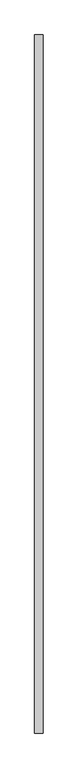
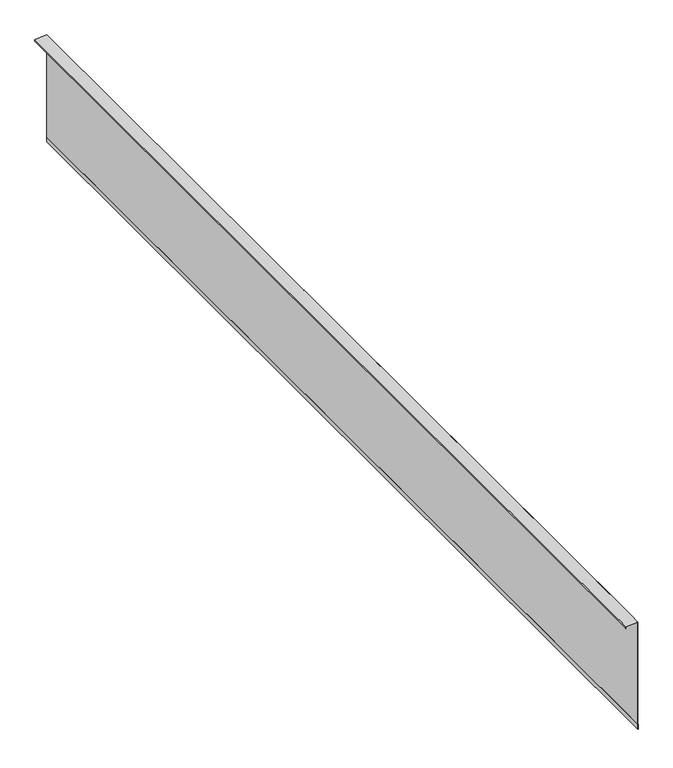
"""IFC4 building model written with IfcOpenShell, lengths in millimetres: proxy geometry, Generic Models 7:Generic Models 1:5:Generic Models 1:5 : Generic Models 7:Generic Models 1:337419:28 : Generic Models 7:Generic Models 1:5:Generic Models 1:5 : Generic Models 7:Generic Models 1:337419:311462."""

from ifc_helpers import new_model, si_unit, origin, place, context, project, spatial, faceted_brep, source, transform, mapped, element, save


def generic_models_2a065a63(model_context):
    return source(origin(), model_context, "Body", "Brep", [
        faceted_brep([(579321.2054739, -579015.7726341, 4172.6354866), (579322.7929739, -579015.7726341, 4170.3683016), (579323.5379701, -579015.7726341, 4169.3043368), (579323.5379701, -579015.7726341, 4076.6752754), (579325.1254701, -579015.7726341, 4076.6752754), (579325.1254701, -579015.7726341, 4169.8048737), (579322.7929739, -579015.7726341, 4173.1360234), (579322.7929739, -579015.7726341, 6174.2616872), (579100.5193767, -579015.7726341, 6162.6128216), (579100.5193767, -579015.7726341, 6125.115987), (579102.1068767, -579015.7726341, 6125.115987), (579102.1068767, -579015.7726341, 6161.1063403), (579321.2054739, -579015.7726341, 6172.5888113), (579321.2054741, -560045.1489433, 4172.6354866), (579321.2054741, -560045.1489433, 6172.5888113), (579102.1068769, -560045.1489433, 6161.1063403), (579102.1068769, -560045.1489433, 6125.115987), (579100.5193769, -560045.1489433, 6125.115987), (579100.5193769, -560045.1489433, 6162.6128216), (579322.7929741, -560045.1489433, 6174.2616872), (579322.7929741, -560045.1489433, 4173.1360234), (579325.1254703, -560045.1489433, 4169.8048737), (579325.1254703, -560045.1489433, 4076.6752754), (579323.5379703, -560045.1489433, 4076.6752754), (579323.5379703, -560045.1489433, 4169.3043368), (579322.7929739, -578891.4324161, 6174.2616872), (579322.7929739, -578921.7652908, 6174.2616872), (579322.7929739, -579014.1851341, 6174.2616872), (579321.2054739, -579014.1851341, 4172.6354866), (579321.2054739, -579014.1851341, 6172.5888113), (579321.2054739, -578889.8449161, 6172.5888113), (579321.2054739, -578859.5120415, 6172.5888113), (579102.1068767, -579014.1851341, 6161.1063403), (579102.1068767, -578795.0865368, 6161.1063403), (579102.1068767, -578793.4990368, 6161.1063403), (579102.1068767, -579014.1851341, 6125.115987), (579100.5193767, -579014.1851341, 6125.115987), (579100.5193767, -579014.1851341, 6162.6128216), (579100.5193767, -578795.0865368, 6162.6128216), (579100.5193767, -578793.4990368, 6162.6128216)], [[[0, 1, 2, 3, 4, 5, 6, 7, 8, 9, 10, 11, 12]], [[13, 14, 15, 16, 17, 18, 19, 20, 21, 22, 23, 24]], [[7, 6, 20, 19, 25, 26, 27]], [[6, 5, 21, 20]], [[5, 4, 22, 21]], [[4, 3, 23, 22]], [[3, 2, 24, 23]], [[2, 1, 0, 28, 13, 24]], [[0, 12, 29, 30, 31, 14, 13, 28]], [[12, 11, 32, 33, 34, 15, 14, 31, 30, 29]], [[11, 10, 35, 16, 15, 34, 33, 32]], [[10, 9, 36, 17, 16, 35]], [[9, 8, 37, 38, 39, 18, 17, 36]], [[8, 7, 27, 26, 25, 19, 18, 39, 38, 37]]]),
    ])


if __name__ == "__main__":
    model = new_model("IFC4")
    model_context = context("Model", 3, world=origin())
    ifc_project = project(units=[si_unit("LENGTHUNIT", "METRE", prefix="MILLI")], contexts=[model_context])
    site = spatial("IfcSite", under=ifc_project)
    building = spatial("IfcBuilding", under=site)
    placement = place(None, origin())
    generic_models_shape = generic_models_2a065a63(model_context)
    element("IfcBuildingElementProxy", 1, Name="Generic Models 7:Generic Models 1:5:Generic Models 1:5 : Generic Models 7:Generic Models 1:337419:28 : Generic Models 7:Generic Models 1:5:Generic Models 1:5 : Generic Models 7:Generic Models 1:337419:311462", ObjectType="Generic Models 7:Generic Models 1:5:Generic Models 1:5 : Generic Models 7:Generic Models 1:337419:28 : Generic Models 7:Generic Models 1:5:Generic Models 1:5 : Generic Models 7:Generic Models 1:337419:311462", at=placement, inside=building, context=model_context, shape_type="MappedRepresentation", body=[
        mapped(generic_models_shape, transform((0.0, 0.0, 0.0), x_axis=(1.0, 0.0, 0.0), y_axis=(0.0, 1.0, 0.0), z_axis=(0.0, 0.0, 1.0))),
    ])
    save(model, "model.ifc")

# Revit data of these elements
# Type "Generic Models 7:Generic Models 1:5:Generic Models 1:5 : Generic Models 7:Generic Models 1:337419:28 : Generic Models 7:Generic Models 1:5:Generic Models 1:5 : Generic Models 7:Generic Models 1:337419:311462"
#   NameOverride = "Generic Models 7:Generic Models 1:5:Generic Models 1:5 : Generic Models 7:Generic Models 1:337419:311462"
#   ObjectTypeOverride = "Generic Models 1:5 : Generic Models 7:Generic Models 1:337419"
#   Reference = "Generic Models 1"
#   Tag = "311462"
# Element 1 (IfcBuildingElementProxy, "Generic Models 7:Generic Models 1:5:Generic Models 1:5 : Generic Models 7:Generic Models 1:337419:28 : Generic Models 7:Generic Models 1:5:Generic Models 1:5 : Generic Models 7:Generic Models 1:337419:311462")
#   Materials on its faces: "UV STABLE WATER RESISTANT VAPOR PERMEABLE AIR BARRIER (WRB) - WRAP JAMBS/HEADERS - BLACK COLOR"
# Materials
#   "UV STABLE WATER RESISTANT VAPOR PERMEABLE AIR BARRIER (WRB) - WRAP JAMBS/HEADERS - BLACK COLOR": class "Generic", colour RGB 51 162 45, transparency 0, Description = "Polyethylene film membrane", Cost = 0
